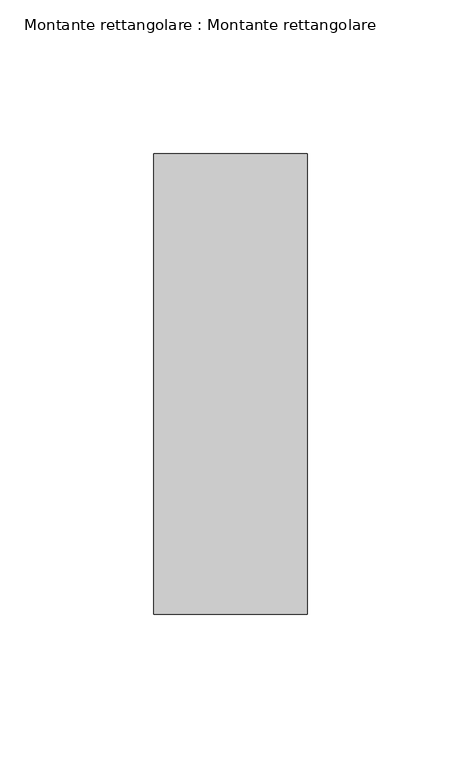
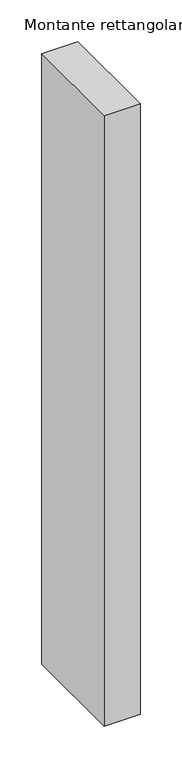
"""IFC4 building model written with IfcOpenShell, lengths in millimetres: member geometry, Montante rettangolare : Montante rettangolare."""

from ifc_helpers import new_model, si_unit, frame, origin, place, context, project, spatial, polyline, outline, extrude, source, transform, mapped, element, save


def montante_rettangolare_montante_rettangolare_060a51f6(model_context):
    return source(origin(), model_context, "Body", "SweptSolid", [
        extrude(outline(polyline([(0.0, 75.0), (0.0, -75.0), (-50.0, -75.0), (-50.0, 75.0), (0.0, 75.0)])), frame((0.0, 0.0, -895.0), z_axis=(0.0, 0.0, 1.0), x_axis=(1.0, 0.0, 0.0)), (0.0, 0.0, 1.0), 895.0),
    ])


if __name__ == "__main__":
    model = new_model("IFC4")
    model_context = context("Model", 3, world=origin())
    ifc_project = project(units=[si_unit("LENGTHUNIT", "METRE", prefix="MILLI")], contexts=[model_context])
    site = spatial("IfcSite", under=ifc_project)
    building = spatial("IfcBuilding", under=site)
    placement = place(None, origin())
    montante_rettangolare_montante_rettangolare_shape = montante_rettangolare_montante_rettangolare_060a51f6(model_context)
    element("IfcMember", 1, ObjectType="Montante rettangolare : Montante rettangolare", at=placement, inside=building, context=model_context, shape_type="MappedRepresentation", body=[
        mapped(montante_rettangolare_montante_rettangolare_shape, transform((0.0, 0.0, 0.0), x_axis=(1.0, 0.0, 0.0), y_axis=(0.0, 1.0, 0.0), z_axis=(0.0, 0.0, 1.0))),
    ])
    save(model, "model.ifc")

# Revit data of these elements
# Type "Montante rettangolare : Montante rettangolare"
#   built-in parameter 1007304 = 0.492126 (stored number, unit not read)
#   built-in parameter 1007301 = 0.082021 (stored number, unit not read)
#   built-in parameter 1007300 = 0.082021 (stored number, unit not read)
# Element 1 (IfcMember, "Montante rettangolare : Montante rettangolare")
#   Materials on its faces: "Acciaio"
# Materials
#   "Acciaio": class "Metallo", colour RGB 247 247 247, transparency 0, Description = "Acciaio, finitura zigrinata", Cost = 0
